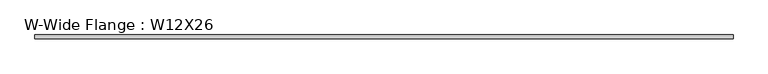
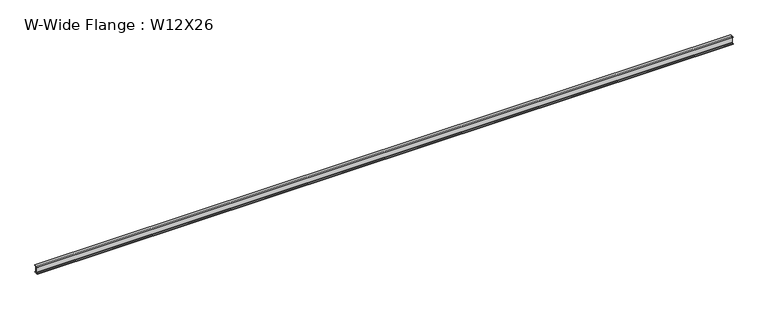
"""IFC4 building model written with IfcOpenShell, lengths in millimetres: beam geometry, W-Wide Flange : W12X26."""

from ifc_helpers import new_model, si_unit, point, frame, frame_2d, origin, place, context, project, spatial, polyline, circle_curve, trimmed, segment, composite_curve, outline, extrude, source, transform, mapped, element, save


def w_wide_flange_w12x26_7742fcc8(model_context):
    return source(origin(), model_context, "Body", "SweptSolid", [
        extrude(outline(composite_curve([segment(polyline([(82.4011719, -145.5539063), (82.4011719, -155.178125), (-82.4011719, -155.178125), (-82.4011719, -145.5539063), (-20.2902344, -145.5539063)]), True, "CONTINUOUS"), segment(trimmed(circle_curve(frame_2d((-20.2902344, -128.190625)), 17.3632812), [point((-20.2902344, -145.5539063))], [point((-2.9269531, -128.190625))], True, "CARTESIAN"), True, "CONTINUOUS"), segment(polyline([(-2.9269531, -128.190625), (-2.9269531, 128.190625)]), True, "CONTINUOUS"), segment(trimmed(circle_curve(frame_2d((-20.2902344, 128.190625)), 17.3632812), [point((-2.9269531, 128.190625))], [point((-20.2902344, 145.5539062))], True, "CARTESIAN"), True, "CONTINUOUS"), segment(polyline([(-20.2902344, 145.5539062), (-82.4011719, 145.5539062), (-82.4011719, 155.178125), (82.4011719, 155.178125), (82.4011719, 145.5539062), (20.2902344, 145.5539062)]), True, "CONTINUOUS"), segment(trimmed(circle_curve(frame_2d((20.2902344, 128.190625)), 17.3632812), [point((20.2902344, 145.5539062))], [point((2.9269531, 128.190625))], True, "CARTESIAN"), True, "CONTINUOUS"), segment(polyline([(2.9269531, 128.190625), (2.9269531, -128.190625)]), True, "CONTINUOUS"), segment(trimmed(circle_curve(frame_2d((20.2902344, -128.190625)), 17.3632812), [point((2.9269531, -128.190625))], [point((20.2902344, -145.5539063))], True, "CARTESIAN"), True, "CONTINUOUS"), segment(polyline([(20.2902344, -145.5539063), (82.4011719, -145.5539063)]), True, "CONTINUOUS")], self_intersect=False)), frame((-14782.8, 0.0, 0.0), z_axis=(1.0, 0.0, 0.0), x_axis=(0.0, 1.0, 0.0)), (0.0, 0.0, 1.0), 29565.6),
    ])


if __name__ == "__main__":
    model = new_model("IFC4")
    model_context = context("Model", 3, world=origin())
    ifc_project = project(units=[si_unit("LENGTHUNIT", "METRE", prefix="MILLI")], contexts=[model_context])
    site = spatial("IfcSite", under=ifc_project)
    building = spatial("IfcBuilding", under=site)
    placement = place(None, origin())
    w_wide_flange_w12x26_shape = w_wide_flange_w12x26_7742fcc8(model_context)
    element("IfcBeam", 1, ObjectType="W-Wide Flange : W12X26", at=placement, inside=building, context=model_context, shape_type="MappedRepresentation", body=[
        mapped(w_wide_flange_w12x26_shape, transform((0.0, 0.0, 0.0), x_axis=(1.0, 0.0, 0.0), y_axis=(0.0, 1.0, 0.0), z_axis=(0.0, 0.0, 1.0))),
    ])
    save(model, "model.ifc")

# Revit data of these elements
# Type "W-Wide Flange : W12X26"
#   Assembly Code = "B10"
#   W = 26
#   Length [instance default] = 5' - 0"
#   bf = 0' - 6 125/256"
#   d = 1' - 0 7/32"
#   k = 0' - 1 1/16"
#   k2 = 0' - 0 175/256"
#   tf = 0' - 0 97/256"
#   tw = 0' - 0 59/256"
#   A = 0.053125 SF
#   Structural Material [instance default] = none
